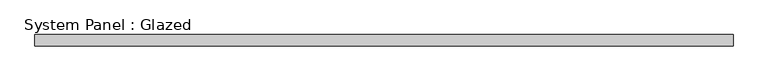
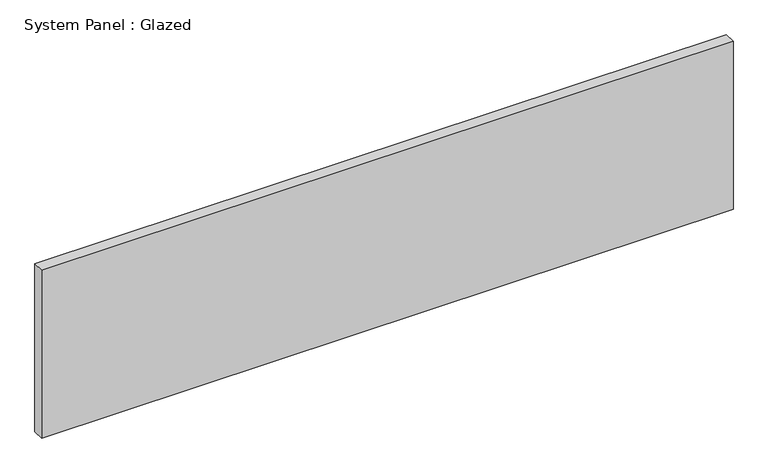
"""IFC4 building model written with IfcOpenShell, lengths in millimetres: plate geometry, System Panel : Glazed."""

from ifc_helpers import new_model, si_unit, origin, origin_with_axes, place, context, project, spatial, polyline, outline, extrude, source, transform, mapped, element, save


def system_panel_glazed_d7984a1f(model_context):
    return source(origin(), model_context, "Body", "SweptSolid", [
        extrude(outline(polyline([(768.3500002, -44.45), (-768.3500002, -44.45), (-768.3500002, -19.05), (768.3500002, -19.05), (768.3500002, -44.45)])), origin_with_axes(), (0.0, 0.0, 1.0), 393.7),
    ])


if __name__ == "__main__":
    model = new_model("IFC4")
    model_context = context("Model", 3, world=origin())
    ifc_project = project(units=[si_unit("LENGTHUNIT", "METRE", prefix="MILLI")], contexts=[model_context])
    site = spatial("IfcSite", under=ifc_project)
    building = spatial("IfcBuilding", under=site)
    placement = place(None, origin())
    system_panel_glazed_shape = system_panel_glazed_d7984a1f(model_context)
    element("IfcPlate", 1, ObjectType="System Panel : Glazed", at=placement, inside=building, context=model_context, shape_type="MappedRepresentation", body=[
        mapped(system_panel_glazed_shape, transform((0.0, 0.0, 0.0), x_axis=(1.0, 0.0, 0.0), y_axis=(0.0, 1.0, 0.0), z_axis=(0.0, 0.0, 1.0))),
    ])
    save(model, "model.ifc")

# Revit data of these elements
# Element 1 (IfcPlate, "System Panel : Glazed")
#   Materials on its faces: "Glass"
# Materials
#   "Glass": class "Glass", colour RGB 0 128 192, transparency 0.75
